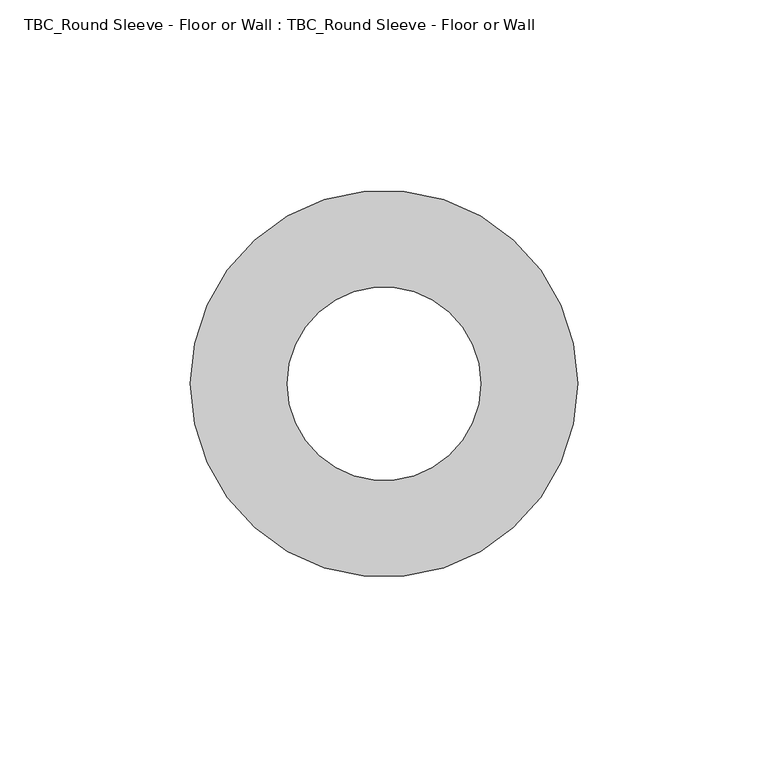
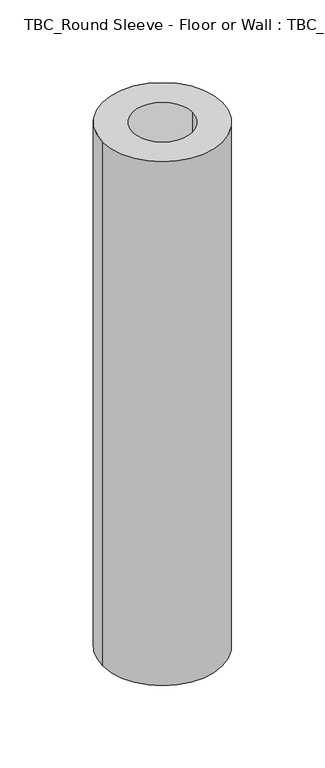
"""IFC4 building model written with IfcOpenShell, lengths in millimetres: proxy geometry, TBC_Round Sleeve - Floor or Wall : TBC_Round Sleeve - Floor or Wall."""

import ifcopenshell
import ifcopenshell.guid

model = None  # the IFC model being written
_history = None  # IfcOwnerHistory: only IFC2X3 demands one
_inside = {}  # id of a spatial element -> (the spatial element, [elements in it])
_under = {}  # id of a project, library or spatial element -> (it, [spatial elements below it])
_declared = {}  # id of a project -> (the project, [libraries it declares])
_typed = {}  # id of a type object -> (the type object, [elements of that type])
_made_of = {}  # id of a material, layer set ... -> (it, [elements and type objects made of it])


def new_model(schema):
    """Start an empty IFC model of exactly this schema.

    Asked for "IFC4X3", IfcOpenShell would pick the latest addendum, in which some entities
    have other attributes; the version numbers below select the first issue.
    IFC2X3 requires an IfcOwnerHistory on every rooted entity: one is made here for all.
    """
    global model, _history
    if schema == "IFC4X3":
        model = ifcopenshell.file(schema_version=(4, 3, 0, 0))
    else:
        model = ifcopenshell.file(schema=schema)
    _inside.clear()
    _under.clear()
    _declared.clear()
    _typed.clear()
    _made_of.clear()
    _history = None
    if model.schema == "IFC2X3":
        org = make("IfcOrganization", Name="unknown")
        user = make(
            "IfcPersonAndOrganization",
            ThePerson=make("IfcPerson", FamilyName="unknown"),
            TheOrganization=org,
        )
        app = make(
            "IfcApplication",
            ApplicationDeveloper=org,
            Version="unknown",
            ApplicationFullName="unknown",
            ApplicationIdentifier="unknown",
        )
        _history = make(
            "IfcOwnerHistory",
            OwningUser=user,
            OwningApplication=app,
            ChangeAction="ADDED",
            CreationDate=0,
        )
    return model


def make(cls, **values):
    """One entity of the class cls with the attributes given. An attribute that is None is left unset."""
    return model.create_entity(
        cls, **{name: value for name, value in values.items() if value is not None}
    )


def rooted(cls, **values):
    """An entity with a GlobalId (a new one), such as an element, a storey or a relation."""
    return make(cls, GlobalId=ifcopenshell.guid.new(), OwnerHistory=_history, **values)


def si_unit(unit_type, name, prefix=None):
    """IfcSIUnit, for example si_unit("LENGTHUNIT", "METRE", prefix="MILLI")."""
    return make("IfcSIUnit", UnitType=unit_type, Prefix=prefix, Name=name)


def assignment(units):
    """IfcUnitAssignment: the units of a project."""
    return None if units is None else make("IfcUnitAssignment", Units=units)


def point(xyz):
    """IfcCartesianPoint."""
    return None if xyz is None else make("IfcCartesianPoint", Coordinates=xyz)


def direction(xyz):
    """IfcDirection."""
    return None if xyz is None else make("IfcDirection", DirectionRatios=xyz)


def frame(location, z_axis=None, x_axis=None):
    """IfcAxis2Placement3D, a coordinate frame: its origin and axes. An axis left out is left unset."""
    return make(
        "IfcAxis2Placement3D",
        Location=point(location),
        Axis=direction(z_axis),
        RefDirection=direction(x_axis),
    )


def frame_2d(location, x_axis=None):
    """IfcAxis2Placement2D, a coordinate frame in the plane: its origin and x axis."""
    return make(
        "IfcAxis2Placement2D", Location=point(location), RefDirection=direction(x_axis)
    )


def origin():
    """The frame at (0, 0, 0) with its axes left unset."""
    return frame((0.0, 0.0, 0.0))


def origin_2d():
    """The frame at (0, 0) in the plane with its x axis left unset."""
    return frame_2d((0.0, 0.0))


def place(relative_to, where):
    """IfcLocalPlacement: puts the frame where relative to a parent placement (None: the world)."""
    return make(
        "IfcLocalPlacement", PlacementRelTo=relative_to, RelativePlacement=where
    )


def context(
    kind, dimensions, precision=None, world=None, true_north=None, identifier=None
):
    """IfcGeometricRepresentationContext, for example the 3D "Model" context."""
    return make(
        "IfcGeometricRepresentationContext",
        ContextIdentifier=identifier,
        ContextType=kind,
        CoordinateSpaceDimension=dimensions,
        Precision=precision,
        WorldCoordinateSystem=world,
        TrueNorth=true_north,
    )


def project(units=None, contexts=None):
    """IfcProject with its units and contexts."""
    return rooted(
        "IfcProject",
        Name="project",
        RepresentationContexts=contexts,
        UnitsInContext=assignment(units),
    )


def spatial(cls, under=None, at=None, **own):
    """A site, building, storey or space (cls), placed at a placement, below another one or the project."""
    s = rooted(cls, ObjectPlacement=at, **own)
    if under is not None:
        _under.setdefault(under.id(), (under, []))[1].append(s)
    return s


def circle_curve(where, radius):
    """IfcCircle in the frame where."""
    return make("IfcCircle", Position=where, Radius=radius)


def trimmed(basis, trim1, trim2, sense, master):
    """IfcTrimmedCurve: the piece of a basis curve between two trims."""
    return make(
        "IfcTrimmedCurve",
        BasisCurve=basis,
        Trim1=trim1,
        Trim2=trim2,
        SenseAgreement=sense,
        MasterRepresentation=master,
    )


def segment(curve, same_sense, transition):
    """IfcCompositeCurveSegment."""
    return make(
        "IfcCompositeCurveSegment",
        Transition=transition,
        SameSense=same_sense,
        ParentCurve=curve,
    )


def composite_curve(segments, self_intersect=None):
    """IfcCompositeCurve: segments joined end to end."""
    return make("IfcCompositeCurve", Segments=segments, SelfIntersect=self_intersect)


def outline(outer, holes=None, kind="AREA"):
    """IfcArbitraryClosedProfileDef: a profile drawn as a closed curve; with holes, ...WithVoids."""
    if holes is None:
        return make("IfcArbitraryClosedProfileDef", ProfileType=kind, OuterCurve=outer)
    return make(
        "IfcArbitraryProfileDefWithVoids",
        ProfileType=kind,
        OuterCurve=outer,
        InnerCurves=holes,
    )


def extrude(swept, where, along, depth):
    """IfcExtrudedAreaSolid: the profile swept, set in the frame where, extruded along a direction by depth."""
    return make(
        "IfcExtrudedAreaSolid",
        SweptArea=swept,
        Position=where,
        ExtrudedDirection=direction(along),
        Depth=depth,
    )


def shape(context_of_items, identifier, shape_type, items):
    """IfcShapeRepresentation: the items that make up one representation, for example the "Body"."""
    return make(
        "IfcShapeRepresentation",
        ContextOfItems=context_of_items,
        RepresentationIdentifier=identifier,
        RepresentationType=shape_type,
        Items=items,
    )


def source(mapping_origin, context_of_items, identifier, shape_type, items):
    """IfcRepresentationMap: a shape defined once, which mapped items show again and again."""
    return make(
        "IfcRepresentationMap",
        MappingOrigin=mapping_origin,
        MappedRepresentation=shape(context_of_items, identifier, shape_type, items),
    )


def transform(
    local_origin,
    x_axis=None,
    y_axis=None,
    z_axis=None,
    scale=None,
    scale2=None,
    scale3=None,
    uniform=True,
):
    """IfcCartesianTransformationOperator3D, or its non-uniform kind. x_axis, y_axis, z_axis: its Axis1, 2, 3."""
    if uniform:
        return make(
            "IfcCartesianTransformationOperator3D",
            Axis1=direction(x_axis),
            Axis2=direction(y_axis),
            LocalOrigin=point(local_origin),
            Scale=scale,
            Axis3=direction(z_axis),
        )
    return make(
        "IfcCartesianTransformationOperator3DnonUniform",
        Axis1=direction(x_axis),
        Axis2=direction(y_axis),
        LocalOrigin=point(local_origin),
        Scale=scale,
        Axis3=direction(z_axis),
        Scale2=scale2,
        Scale3=scale3,
    )


def mapped(mapping_source, mapping_target):
    """IfcMappedItem: shows the shape of a source again, moved by a transform."""
    return make(
        "IfcMappedItem", MappingSource=mapping_source, MappingTarget=mapping_target
    )


def made_of(thing, what):
    """Note that an element or type object is made of a material, layer set ...; save() writes the relation."""
    if what is not None:
        _made_of.setdefault(what.id(), (what, []))[1].append(thing)
    return thing


def element(
    cls,
    number,
    at=None,
    inside=None,
    cuts=None,
    type_object=None,
    material=None,
    context=None,
    identifier="Body",
    shape_type=None,
    held_by="IfcProductDefinitionShape",
    body=None,
    shapes=None,
    **own,
):
    """One element of the class cls, such as IfcWall. Its Tag is "e" and its number.

    at: its placement. inside: the storey or other place that contains it. cuts: it is an
    opening in that element (IfcRelVoidsElement). A single representation is given by context,
    identifier, shape_type and body (its items); several are given by shapes. held_by: the class
    of the entity that holds the representations. save() writes the other relations.
    """
    e = rooted(cls, Tag="e%d" % number, ObjectPlacement=at, **own)
    if body is not None:
        shapes = [shape(context, identifier, shape_type, body)]
    if shapes is not None:
        e.Representation = make(held_by, Representations=shapes)
    if inside is not None:
        _inside.setdefault(inside.id(), (inside, []))[1].append(e)
    if cuts is not None:
        rooted(
            "IfcRelVoidsElement", RelatingBuildingElement=cuts, RelatedOpeningElement=e
        )
    if type_object is not None:
        _typed.setdefault(type_object.id(), (type_object, []))[1].append(e)
    return made_of(e, material)


def aggregate(whole, parts):
    """IfcRelAggregates: a whole, such as a stair, and the parts it consists of."""
    return rooted("IfcRelAggregates", RelatingObject=whole, RelatedObjects=parts)


def save(model, path):
    """Write the relations noted so far, then the file.

    IfcRelAggregates (storeys below a building ...), IfcRelContainedInSpatialStructure (elements
    in a storey), IfcRelDefinesByType, IfcRelAssociatesMaterial and IfcRelDeclares: one each for
    every whole, place, type object, material and project.
    """
    for whole, parts in _under.values():
        aggregate(whole, parts)
    for where, things in _inside.values():
        rooted(
            "IfcRelContainedInSpatialStructure",
            RelatedElements=things,
            RelatingStructure=where,
        )
    for kind, things in _typed.values():
        rooted("IfcRelDefinesByType", RelatedObjects=things, RelatingType=kind)
    for what, things in _made_of.values():
        rooted("IfcRelAssociatesMaterial", RelatedObjects=things, RelatingMaterial=what)
    for by, libraries in _declared.values():
        rooted("IfcRelDeclares", RelatingContext=by, RelatedDefinitions=libraries)
    model.write(path)


def tbc_round_sleeve_floor_or_wall_tbc_round_sleeve_floor_or_5e24f8f3(model_context):
    return source(origin(), model_context, "Body", "SweptSolid", [
        extrude(outline(composite_curve([segment(trimmed(circle_curve(origin_2d(), 50.8), [point((-50.8, 0.0))], [point((50.8, 0.0))], False, "CARTESIAN"), True, "CONTINUOUS"), segment(trimmed(circle_curve(origin_2d(), 50.8), [point((50.8, 0.0))], [point((-50.8, 0.0))], False, "CARTESIAN"), True, "CONTINUOUS")], self_intersect=False), holes=[composite_curve([segment(trimmed(circle_curve(origin_2d(), 25.4), [point((-25.4, 0.0))], [point((25.4, 0.0))], True, "CARTESIAN"), True, "CONTINUOUS"), segment(trimmed(circle_curve(origin_2d(), 25.4), [point((25.4, 0.0))], [point((-25.4, 0.0))], True, "CARTESIAN"), True, "CONTINUOUS")], self_intersect=False)]), frame((0.0, 0.0, -469.9), z_axis=(0.0, 0.0, 1.0), x_axis=(1.0, 0.0, 0.0)), (0.0, 0.0, 1.0), 469.9),
    ])


if __name__ == "__main__":
    model = new_model("IFC4")
    model_context = context("Model", 3, world=origin())
    ifc_project = project(units=[si_unit("LENGTHUNIT", "METRE", prefix="MILLI")], contexts=[model_context])
    site = spatial("IfcSite", under=ifc_project)
    building = spatial("IfcBuilding", under=site)
    placement = place(None, origin())
    tbc_round_sleeve_floor_or_wall_tbc_round_sleeve_floor_or_shape = tbc_round_sleeve_floor_or_wall_tbc_round_sleeve_floor_or_5e24f8f3(model_context)
    element("IfcBuildingElementProxy", 1, Name="TBC_Round Sleeve - Floor or Wall : TBC_Round Sleeve - Floor or Wall", ObjectType="TBC_Round Sleeve - Floor or Wall : TBC_Round Sleeve - Floor or Wall", at=placement, inside=building, context=model_context, shape_type="MappedRepresentation", body=[
        mapped(tbc_round_sleeve_floor_or_wall_tbc_round_sleeve_floor_or_shape, transform((0.0, 0.0, 0.0), x_axis=(1.0, 0.0, 0.0), y_axis=(0.0, 1.0, 0.0), z_axis=(0.0, 0.0, 1.0))),
    ])
    save(model, "model.ifc")

# Revit data of these elements
# Type "TBC_Round Sleeve - Floor or Wall : TBC_Round Sleeve - Floor or Wall"
#   Tag Dimension [instance default] = ""
#   MEP Type [instance default] = ""
#   MEP Element [instance default] = ""
#   MEP Category [instance default] = ""
#   Host Element Type [instance default] = ""
#   Host Element Id [instance default] = ""
#   Host Element Category [instance default] = ""
#   Control Line Y [instance default] = ""
#   Control Line X [instance default] = ""
#   Sleeve Radius [instance default] = 1' - 0"
#   Sleeve Edge [instance default] = 1' - 2"
#   Sleeve Depth [instance default] = 3' - 0"
#   Distance Y [instance default] = 0' - 0"
#   Distance X [instance default] = 0' - 0"
#   Default Elevation = 0
# Element 1 (IfcBuildingElementProxy, "TBC_Round Sleeve - Floor or Wall : TBC_Round Sleeve - Floor or Wall")
#   Tag Dimension = "2\"ø"
#   MEP Type = "PLG-G"
#   MEP Element = "898860"
#   MEP Category = "Pipe"
#   Host Element Type = "Roof Plank-Sleeves"
#   Host Element Id = "1525183"
#   Host Element Category = "Floors"
#   Sleeve Radius = 0' - 2"
#   Sleeve Edge = 0' - 4"
#   Sleeve Depth = 1' - 6 1/2"
